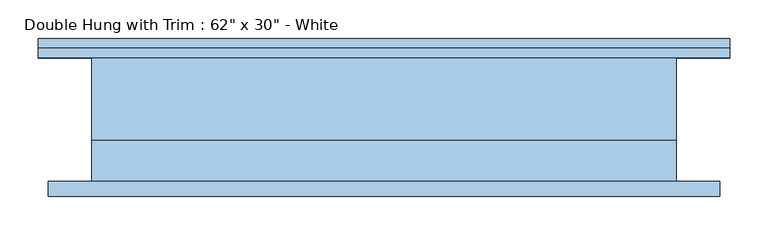
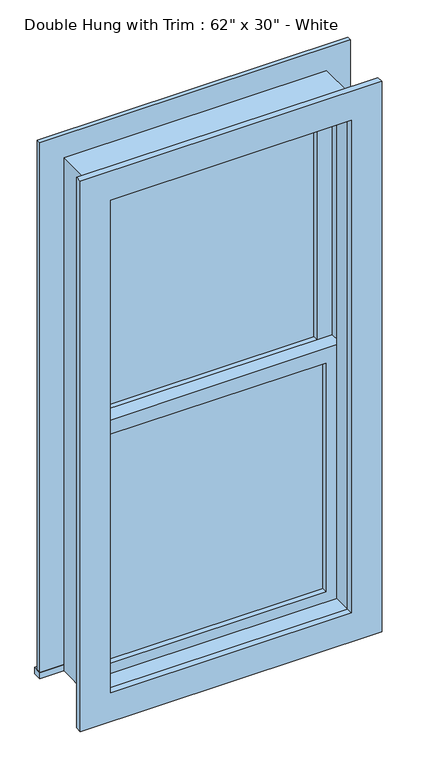
"""IFC4 building model written with IfcOpenShell, lengths in millimetres: window geometry."""

from ifc_helpers import new_model, si_unit, frame, origin, place, context, project, spatial, polyline, outline, extrude, source, transform, mapped, element, save


def window_3e11be29(model_context):
    return source(origin(), model_context, "Body", "SweptSolid", [
        extrude(outline(polyline([(-317.5, 1.5875), (317.5, 1.5875), (317.5, -11.1125), (-317.5, -11.1125), (-317.5, 1.5875)])), frame((0.0, 0.0, 977.9), z_axis=(0.0, 0.0, 1.0), x_axis=(1.0, 0.0, 0.0)), (0.0, 0.0, 1.0), 701.675),
        extrude(outline(polyline([(1724.025, -361.95), (933.45, -361.95), (933.45, 361.95), (1724.025, 361.95), (1724.025, -361.95)]), holes=[polyline([(1679.575, -317.5), (1679.575, 317.5), (977.9, 317.5), (977.9, -317.5), (1679.575, -317.5)])]), frame((0.0, -26.9875, 0.0), z_axis=(0.0, 1.0, 0.0), x_axis=(0.0, 0.0, 1.0)), (0.0, 0.0, 1.0), 44.45),
        extrude(outline(polyline([(-450.85, 106.3625), (450.85, 106.3625), (450.85, 80.9625), (-450.85, 80.9625), (-450.85, 106.3625)])), frame((0.0, 0.0, 914.4), z_axis=(0.0, 0.0, 1.0), x_axis=(1.0, 0.0, 0.0)), (0.0, 0.0, 1.0), 19.05),
        extrude(outline(polyline([(2470.15, -361.95), (2470.15, 361.95), (933.45, 361.95), (933.45, 450.85), (2559.05, 450.85), (2559.05, -450.85), (933.45, -450.85), (933.45, -361.95), (2470.15, -361.95)])), frame((0.0, 80.9625, 0.0), z_axis=(0.0, 1.0, 0.0), x_axis=(0.0, 0.0, 1.0)), (0.0, 0.0, 1.0), 12.7),
        extrude(outline(polyline([(2546.35, 438.15), (2546.35, -438.15), (857.25, -438.15), (857.25, 438.15), (2546.35, 438.15)]), holes=[polyline([(2457.45, 349.25), (946.15, 349.25), (946.15, -349.25), (2457.45, -349.25), (2457.45, 349.25)])]), frame((0.0, -100.0125, 0.0), z_axis=(0.0, 1.0, 0.0), x_axis=(0.0, 0.0, 1.0)), (0.0, 0.0, 1.0), 19.05),
        extrude(outline(polyline([(317.5, 33.3375), (-317.5, 33.3375), (-317.5, 46.0375), (317.5, 46.0375), (317.5, 33.3375)])), frame((0.0, 0.0, 1724.025), z_axis=(0.0, 0.0, 1.0), x_axis=(1.0, 0.0, 0.0)), (0.0, 0.0, 1.0), 701.675),
        extrude(outline(polyline([(2470.15, -361.95), (1679.575, -361.95), (1679.575, 361.95), (2470.15, 361.95), (2470.15, -361.95)]), holes=[polyline([(2425.7, -317.5), (2425.7, 317.5), (1724.025, 317.5), (1724.025, -317.5), (2425.7, -317.5)])]), frame((0.0, 17.4625, 0.0), z_axis=(0.0, 1.0, 0.0), x_axis=(0.0, 0.0, 1.0)), (0.0, 0.0, 1.0), 44.45),
        extrude(outline(polyline([(2489.2, -381.0), (914.4, -381.0), (914.4, 381.0), (2489.2, 381.0), (2489.2, -381.0)]), holes=[polyline([(2457.45, -349.25), (2457.45, 349.25), (946.15, 349.25), (946.15, -349.25), (2457.45, -349.25)])]), frame((0.0, -80.9625, 0.0), z_axis=(0.0, 1.0, 0.0), x_axis=(0.0, 0.0, 1.0)), (0.0, 0.0, 1.0), 53.975),
        extrude(outline(polyline([(2489.2, 381.0), (2489.2, -381.0), (914.4, -381.0), (914.4, 381.0), (2489.2, 381.0)]), holes=[polyline([(2470.15, 361.95), (933.45, 361.95), (933.45, -361.95), (2470.15, -361.95), (2470.15, 361.95)])]), frame((0.0, -26.9875, 0.0), z_axis=(0.0, 1.0, 0.0), x_axis=(0.0, 0.0, 1.0)), (0.0, 0.0, 1.0), 107.95),
    ])


if __name__ == "__main__":
    model = new_model("IFC4")
    model_context = context("Model", 3, world=origin())
    ifc_project = project(units=[si_unit("LENGTHUNIT", "METRE", prefix="MILLI")], contexts=[model_context])
    site = spatial("IfcSite", under=ifc_project)
    building = spatial("IfcBuilding", under=site)
    placement = place(None, origin())
    window_shape = window_3e11be29(model_context)
    element("IfcWindow", 1, ObjectType="Double Hung with Trim : 62\" x 30\" - White", at=placement, inside=building, context=model_context, shape_type="MappedRepresentation", body=[
        mapped(window_shape, transform((0.0, 0.0, 0.0), x_axis=(1.0, 0.0, 0.0), y_axis=(0.0, 1.0, 0.0), z_axis=(0.0, 0.0, 1.0))),
    ])
    save(model, "model.ifc")

# Revit data of these elements
# Type "Double Hung with Trim : 62\" x 30\" - White"
#   Type Mark = "20"
#   COBie.Type.CreatedBy = "doug.wood@us.ibm.com"
#   COBie.Type.CreatedOn = "2016-04-14T02:07:26"
#   COBie.Type.Name = "Windows_Double Hung with Trim_62\" x 30\"_20"
#   COBie.Type.Category = "23-30 20 17 17 14 : Double-Hung Windows"
#   COBie.Type.Description = "Double Hung with Trim_62\" x 30\""
#   COBie.Type.Manufacturer = ""
#   COBie.Type.ModelNumber = ""
#   Construction Type Id = "GSP4R"
#   Assembly Code = "B2020100"
#   Analytic Construction = "1/8 in Pilkington single glazing"
#   COBie.Type.ReplacementCost = 0
#   Visual Light Transmittance = 0.9
#   Solar Heat Gain Coefficient = 0.78
#   Heat Transfer Coefficient (U) = 3.6886 W/(m²·K)
#   Height = 5' - 2"
#   Default Sill Height = 3' - 0"
#   Trim Projection - Ext. = 0' - 0 1/2"
#   Trim Projection - Int. = 0' - 0 3/4"
#   Trim Width - Exterior = 0' - 3 1/2"
#   Trim Width - Interior = 0' - 3 1/2"
#   Width = 2' - 6"
#   Window Inset = 0' - 0 3/4"
#   COBie.Type = no
#   Glass Pane Material = Glass
#   Sash Material = Sash - White
#   Trim Exterior Material = Trim - White
#   Trim Interior Material = Trim - White
#   Wall Closure = (empty or 0)
# Element 1 (IfcWindow, "Double Hung with Trim : 62\" x 30\" - White")
#   Materials on its faces: "Sash - White", "Trim - White", "Glass"
# Materials
#   "Glass": class "Glass", colour RGB 0 128 192, transparency 0.75, Description = "Soda Lime Glass", Cost = 0
#   "Sash - White": class "Wood", colour RGB 255 255 255, transparency 0, Cost = 0
#   "Trim - White": class "Wood", colour RGB 255 255 255, transparency 0, Cost = 0
